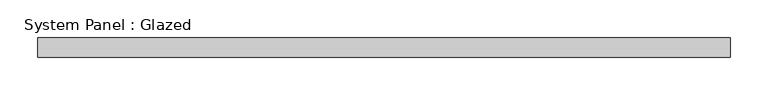
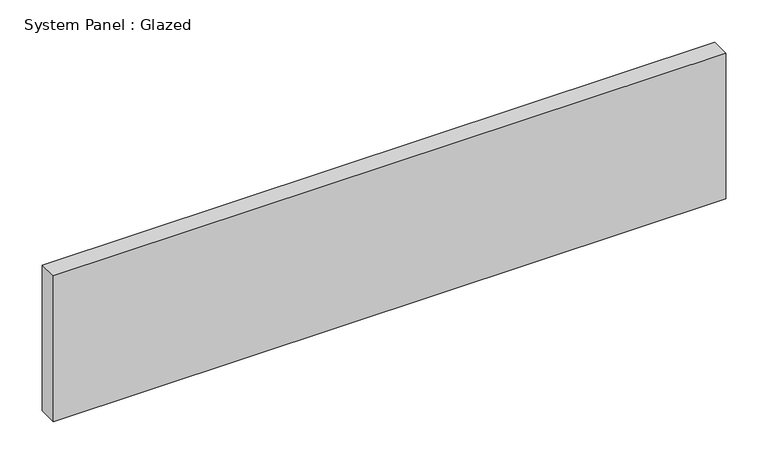
"""IFC4 building model written with IfcOpenShell, lengths in millimetres: plate geometry, System Panel : Glazed."""

from ifc_helpers import new_model, si_unit, origin, origin_with_axes, place, context, project, spatial, polyline, outline, extrude, source, transform, mapped, element, save


def system_panel_glazed_72fe8651(model_context):
    return source(origin(), model_context, "Body", "SweptSolid", [
        extrude(outline(polyline([(457.2, 19.05), (-457.2, 19.05), (-457.2, 44.45), (457.2, 44.45), (457.2, 19.05)])), origin_with_axes(), (0.0, 0.0, 1.0), 209.55),
    ])


if __name__ == "__main__":
    model = new_model("IFC4")
    model_context = context("Model", 3, world=origin())
    ifc_project = project(units=[si_unit("LENGTHUNIT", "METRE", prefix="MILLI")], contexts=[model_context])
    site = spatial("IfcSite", under=ifc_project)
    building = spatial("IfcBuilding", under=site)
    placement = place(None, origin())
    system_panel_glazed_shape = system_panel_glazed_72fe8651(model_context)
    element("IfcPlate", 1, ObjectType="System Panel : Glazed", at=placement, inside=building, context=model_context, shape_type="MappedRepresentation", body=[
        mapped(system_panel_glazed_shape, transform((0.0, 0.0, 0.0), x_axis=(1.0, 0.0, 0.0), y_axis=(0.0, 1.0, 0.0), z_axis=(0.0, 0.0, 1.0))),
    ])
    save(model, "model.ifc")

# Revit data of these elements
# Element 1 (IfcPlate, "System Panel : Glazed")
#   Materials on its faces: "Glass"
# Materials
#   "Glass": class "Glass", colour RGB 0 128 192, transparency 0.75
